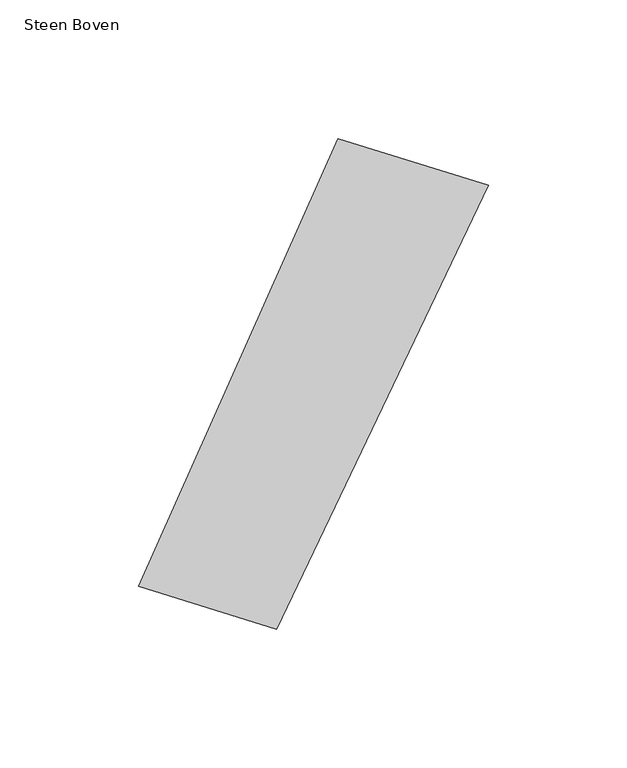
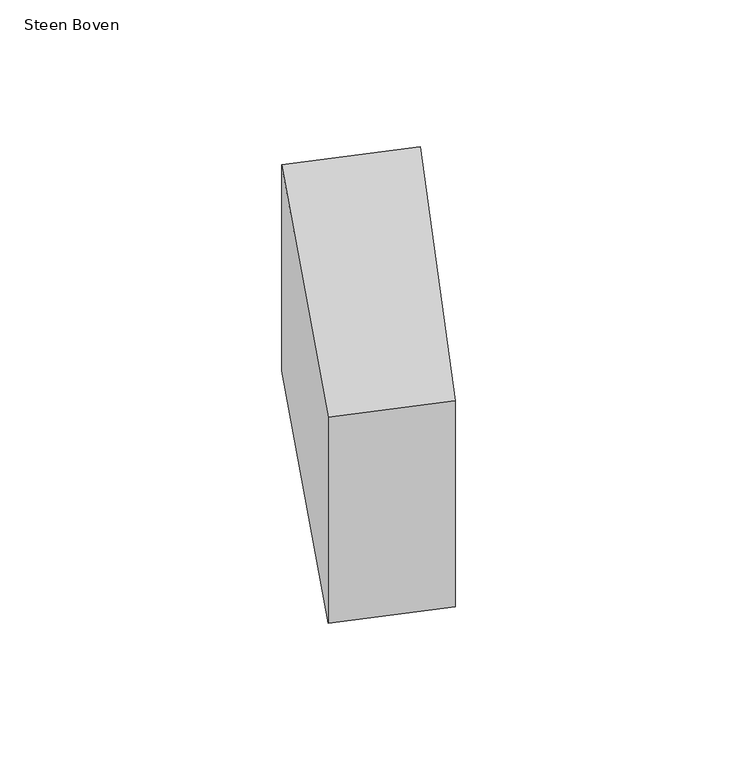
"""IFC4 building model written with IfcOpenShell, lengths in millimetres: proxy geometry, 00_GMA_steen_versie_4 : Steen Boven."""

from ifc_helpers import new_model, si_unit, origin, origin_with_axes, place, context, project, spatial, polyline, outline, extrude, source, transform, mapped, element, save


def steen_boven_789d2b01(model_context):
    return source(origin(), model_context, "Body", "SweptSolid", [
        extrude(outline(polyline([(139.9280508, 152.1762293), (63.7754104, -7.5203255), (14.0953034, 7.8264796), (85.7811753, 168.8863157), (139.9280508, 152.1762293)])), origin_with_axes(), (0.0, 0.0, 1.0), 100.0),
    ])


if __name__ == "__main__":
    model = new_model("IFC4")
    model_context = context("Model", 3, world=origin())
    ifc_project = project(units=[si_unit("LENGTHUNIT", "METRE", prefix="MILLI")], contexts=[model_context])
    site = spatial("IfcSite", under=ifc_project)
    building = spatial("IfcBuilding", under=site)
    placement = place(None, origin())
    steen_boven_shape = steen_boven_789d2b01(model_context)
    element("IfcBuildingElementProxy", 1, Name="00_GMA_steen_versie_4 : Steen Boven", ObjectType="00_GMA_steen_versie_4 : Steen Boven", at=placement, inside=building, context=model_context, shape_type="MappedRepresentation", body=[
        mapped(steen_boven_shape, transform((0.0, 0.0, 0.0), x_axis=(1.0, 0.0, 0.0), y_axis=(0.0, 1.0, 0.0), z_axis=(0.0, 0.0, 1.0))),
    ])
    save(model, "model.ifc")

# Revit data of these elements
# Type "00_GMA_steen_versie_4 : Steen Boven"
#   StootVoegHalfBoven [instance default] = 5 mm
#   StootVoegHalf [instance default] = 5 mm
#   StootVoegBreedteOnder = 10 mm
#   StootVoegBreedteBoven = 10 mm
#   Steendikte = 100 mm
#   LintVoegOnderHalf = 5 mm
#   LintVoegOnder = 10 mm
#   LintVoegBovenHalf = 0 mm
#   LintVoegBoven = 0 mm
#   materiaal = none
#   MateriaalVoeg = none
#   Default Elevation = 0
